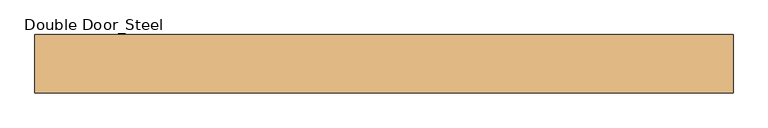
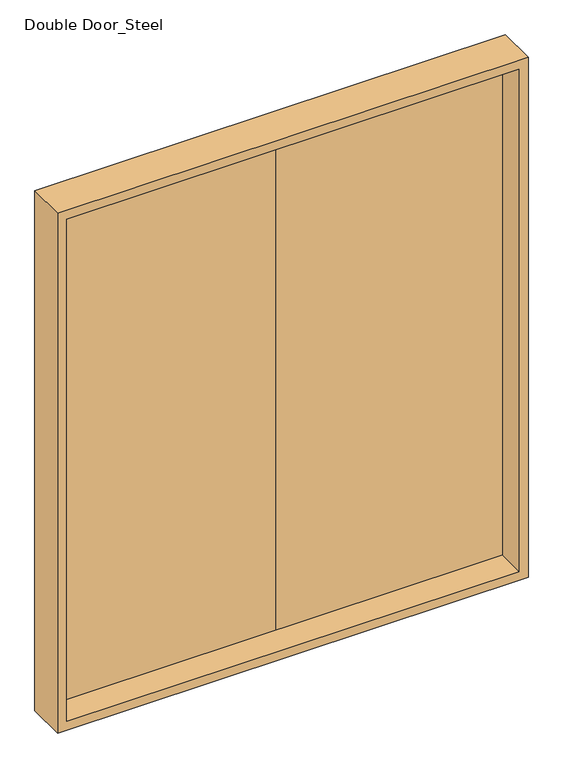
"""IFC4 building model written with IfcOpenShell, lengths in millimetres: door geometry, Double Door_Steel : H_DR_AR_B12_Double Door_Steel_W2000xH2100."""

from ifc_helpers import new_model, si_unit, frame, origin, place, context, project, spatial, polyline, outline, extrude, faceted_brep, source, transform, mapped, element, save


def double_door_steel_580823b0(model_context):
    return source(origin(), model_context, "Body", "SolidModel", [
        extrude(outline(polyline([(880.0, 35.0), (0.0, 35.0), (0.0, 75.0), (880.0, 75.0), (880.0, 35.0)])), frame((0.0, 0.0, 20.0), z_axis=(0.0, 0.0, 1.0), x_axis=(1.0, 0.0, 0.0)), (0.0, 0.0, 1.0), 2060.0),
        extrude(outline(polyline([(0.0, 35.0), (-880.0, 35.0), (-880.0, 75.0), (0.0, 75.0), (0.0, 35.0)])), frame((0.0, 0.0, 20.0), z_axis=(0.0, 0.0, 1.0), x_axis=(1.0, 0.0, 0.0)), (0.0, 0.0, 1.0), 2060.0),
        faceted_brep([(900.0, -75.0, 2100.0), (900.0, 75.0, 2100.0), (-900.0, 75.0, 2100.0), (-900.0, -75.0, 2100.0), (865.0, 35.0, 2065.0), (865.0, -75.0, 2065.0), (-865.0, -75.0, 2065.0), (-865.0, 35.0, 2065.0), (880.0, 75.0, 2080.0), (880.0, 35.0, 2080.0), (-880.0, 35.0, 2080.0), (-880.0, 75.0, 2080.0), (-900.0, 75.0, 0.0), (-900.0, -75.0, 0.0), (-865.0, -75.0, 35.0), (-865.0, 35.0, 35.0), (-880.0, 35.0, 20.0), (-880.0, 75.0, 20.0), (900.0, 75.0, 0.0), (880.0, 75.0, 20.0), (900.0, -75.0, 0.0), (865.0, -75.0, 35.0), (865.0, 35.0, 35.0), (880.0, 35.0, 20.0)], [[[0, 1, 2, 3]], [[4, 5, 6, 7]], [[8, 9, 10, 11]], [[3, 2, 12, 13]], [[7, 6, 14, 15]], [[11, 10, 16, 17]], [[18, 12, 2, 1], [8, 11, 17, 19]], [[13, 12, 18, 20]], [[0, 3, 13, 20], [21, 14, 6, 5]], [[15, 14, 21, 22]], [[23, 16, 10, 9], [4, 7, 15, 22]], [[17, 16, 23, 19]], [[20, 18, 1, 0]], [[22, 21, 5, 4]], [[19, 23, 9, 8]]]),
    ])


if __name__ == "__main__":
    model = new_model("IFC4")
    model_context = context("Model", 3, world=origin())
    ifc_project = project(units=[si_unit("LENGTHUNIT", "METRE", prefix="MILLI")], contexts=[model_context])
    site = spatial("IfcSite", under=ifc_project)
    building = spatial("IfcBuilding", under=site)
    placement = place(None, origin())
    double_door_steel_shape = double_door_steel_580823b0(model_context)
    element("IfcDoor", 1, ObjectType="Double Door_Steel : H_DR_AR_B12_Double Door_Steel_W2000xH2100", at=placement, inside=building, context=model_context, shape_type="MappedRepresentation", body=[
        mapped(double_door_steel_shape, transform((0.0, 0.0, 0.0), x_axis=(1.0, 0.0, 0.0), y_axis=(0.0, 1.0, 0.0), z_axis=(0.0, 0.0, 1.0))),
    ])
    save(model, "model.ifc")

# Revit data of these elements
# Type "Double Door_Steel : H_DR_AR_B12_Double Door_Steel_W2000xH2100"
#   Type Mark = ""
#   프레임 = ""
#   철물 = ""
#   유리/마감 = ""
#   위치/개소 = ""
#   부호 = "1/SD"
#   문번호 = ""
#   문기호 = "SD"
#   Analytic Construction = "<None>"
#   Height = 2100 mm
#   Width = 1800 mm
#   Define Thermal Properties by = 1
#   문 틀 = none
#   문 = none
#   Function = (empty or 0)
#   Assembly Code = ""
#   Wall Closure = (empty or 0)
